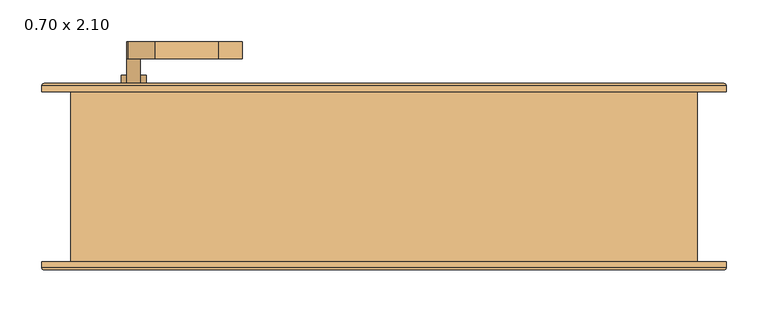
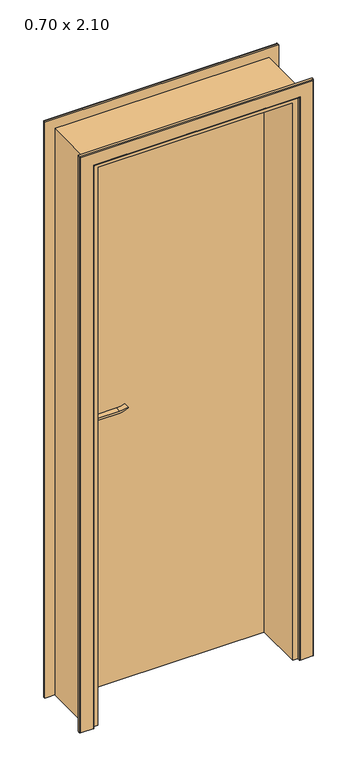
"""IFC4 building model written with IfcOpenShell, lengths in millimetres: door geometry, .CC_ND 300_PORTA SIMPLES DE ABRIR_COM EXTENSÃO : 0.70 x 2.10."""

from ifc_helpers import new_model, si_unit, point, frame, frame_2d, origin, origin_with_axes, place, context, project, spatial, polyline, circle_curve, ellipse_curve, trimmed, segment, composite_curve, outline, extrude, faceted_brep, source, transform, mapped, element, save
from ifc_brep_helpers import plane_surface, cylinder_surface, advanced_brep


def door_0_70_x_2_10_de0bd01c(model_context):
    return source(origin(), model_context, "Body", "SolidModel", [
        extrude(outline(composite_curve([segment(trimmed(circle_curve(frame_2d((964.5, -300.0)), 15.0), [point((964.5, -285.0))], [point((964.5, -315.0))], False, "CARTESIAN"), True, "CONTINUOUS"), segment(trimmed(circle_curve(frame_2d((964.5, -300.0)), 15.0), [point((964.5, -315.0))], [point((964.5, -285.0))], False, "CARTESIAN"), True, "CONTINUOUS")], self_intersect=False)), frame((0.0, 126.4, 0.0), z_axis=(0.0, 1.0, 0.0), x_axis=(0.0, 0.0, 1.0)), (0.0, 0.0, 1.0), 10.0),
        extrude(outline(composite_curve([segment(trimmed(circle_curve(frame_2d((964.5, -300.0)), 15.0), [point((964.5, -285.0))], [point((964.5, -315.0))], False, "CARTESIAN"), True, "CONTINUOUS"), segment(trimmed(circle_curve(frame_2d((964.5, -300.0)), 15.0), [point((964.5, -315.0))], [point((964.5, -285.0))], False, "CARTESIAN"), True, "CONTINUOUS")], self_intersect=False)), frame((0.0, 66.4, 0.0), z_axis=(0.0, 1.0, 0.0), x_axis=(0.0, 0.0, 1.0)), (0.0, 0.0, 1.0), 10.0),
        extrude(outline(composite_curve([segment(trimmed(circle_curve(frame_2d((1024.5, -300.0)), 8.0), [point((1029.1523287, -306.5081363))], [point((1024.5, -292.0))], False, "CARTESIAN"), True, "CONTINUOUS"), segment(trimmed(circle_curve(frame_2d((1019.3738613, -274.6138099)), 18.1261387), [point((1024.5, -292.0))], [point((1037.5, -274.6138099))], True, "CARTESIAN"), True, "CONTINUOUS"), segment(polyline([(1037.5, -274.6138099), (1037.5, -198.3564091)]), True, "CONTINUOUS"), segment(trimmed(circle_curve(frame_2d((1096.7709207, -201.9396612)), 59.3791355), [point((1037.5, -198.3564091))], [point((1046.7135558, -170.0))], False, "CARTESIAN"), True, "CONTINUOUS"), segment(polyline([(1046.7135558, -170.0), (1049.5, -170.0)]), True, "CONTINUOUS"), segment(trimmed(circle_curve(frame_2d((1127.7850638, -198.4227909)), 83.2850902), [point((1049.5, -170.0))], [point((1044.5, -198.3564091))], True, "CARTESIAN"), True, "CONTINUOUS"), segment(polyline([(1044.5, -198.3564091), (1044.5, -274.6325667)]), True, "CONTINUOUS"), segment(trimmed(circle_curve(frame_2d((1007.2555521, -276.3324871)), 37.2832219), [point((1044.5, -274.6325667))], [point((1029.1523287, -306.5081363))], False, "CARTESIAN"), True, "CONTINUOUS")], self_intersect=False)), frame((0.0, 156.4, 0.0), z_axis=(0.0, 1.0, 0.0), x_axis=(0.0, 0.0, 1.0)), (0.0, 0.0, 1.0), 20.0),
        extrude(outline(composite_curve([segment(trimmed(circle_curve(frame_2d((1019.3738682, -274.6138122)), 18.1261318), [point((1024.4999903, -292.0))], [point((1037.5, -274.6138122))], True, "CARTESIAN"), True, "CONTINUOUS"), segment(polyline([(1037.5, -274.6138122), (1037.5, -198.3564091)]), True, "CONTINUOUS"), segment(trimmed(circle_curve(frame_2d((1096.7709207, -201.9396612)), 59.3791355), [point((1037.5, -198.3564091))], [point((1046.7135558, -170.0))], False, "CARTESIAN"), True, "CONTINUOUS"), segment(polyline([(1046.7135558, -170.0), (1049.5, -170.0)]), True, "CONTINUOUS"), segment(trimmed(circle_curve(frame_2d((1127.7850638, -198.4227909)), 83.2850902), [point((1049.5, -170.0))], [point((1044.5, -198.3564091))], True, "CARTESIAN"), True, "CONTINUOUS"), segment(polyline([(1044.5, -198.3564091), (1044.5, -274.6325667)]), True, "CONTINUOUS"), segment(trimmed(circle_curve(frame_2d((1007.2555521, -276.3324871)), 37.2832219), [point((1044.5, -274.6325667))], [point((1029.1523287, -306.5081363))], False, "CARTESIAN"), True, "CONTINUOUS"), segment(trimmed(circle_curve(frame_2d((1024.5, -300.0)), 8.0), [point((1029.1523287, -306.5081363))], [point((1024.4999903, -292.0))], False, "CARTESIAN"), True, "CONTINUOUS")], self_intersect=False)), frame((0.0, 26.4, 0.0), z_axis=(0.0, 1.0, 0.0), x_axis=(0.0, 0.0, 1.0)), (0.0, 0.0, 1.0), 20.0),
        extrude(outline(composite_curve([segment(trimmed(circle_curve(frame_2d((1024.5, -300.0)), 8.0), [point((1024.5, -292.0))], [point((1024.5, -308.0))], False, "CARTESIAN"), True, "CONTINUOUS"), segment(trimmed(circle_curve(frame_2d((1024.5, -300.0)), 8.0), [point((1024.5, -308.0))], [point((1024.5, -292.0))], False, "CARTESIAN"), True, "CONTINUOUS")], self_intersect=False)), frame((0.0, 126.4, 0.0), z_axis=(0.0, 1.0, 0.0), x_axis=(0.0, 0.0, 1.0)), (0.0, 0.0, 1.0), 30.0),
        extrude(outline(composite_curve([segment(trimmed(circle_curve(frame_2d((1024.5, -300.0)), 8.0), [point((1024.5, -292.0))], [point((1024.5, -308.0))], False, "CARTESIAN"), True, "CONTINUOUS"), segment(trimmed(circle_curve(frame_2d((1024.5, -300.0)), 8.0), [point((1024.5, -308.0))], [point((1024.5, -292.0))], False, "CARTESIAN"), True, "CONTINUOUS")], self_intersect=False)), frame((0.0, 46.4, 0.0), z_axis=(0.0, 1.0, 0.0), x_axis=(0.0, 0.0, 1.0)), (0.0, 0.0, 1.0), 30.0),
        extrude(outline(composite_curve([segment(trimmed(circle_curve(frame_2d((954.5, -300.0)), 25.0), [point((954.5, -325.0))], [point((954.5, -275.0))], False, "CARTESIAN"), True, "CONTINUOUS"), segment(polyline([(954.5, -275.0), (1024.5, -275.0)]), True, "CONTINUOUS"), segment(trimmed(circle_curve(frame_2d((1024.5, -300.0)), 25.0), [point((1024.5, -275.0))], [point((1024.5, -325.0))], False, "CARTESIAN"), True, "CONTINUOUS"), segment(polyline([(1024.5, -325.0), (954.5, -325.0)]), True, "CONTINUOUS")], self_intersect=False)), frame((0.0, 116.4, 0.0), z_axis=(0.0, 1.0, 0.0), x_axis=(0.0, 0.0, 1.0)), (0.0, 0.0, 1.0), 10.0),
        extrude(outline(composite_curve([segment(trimmed(circle_curve(frame_2d((954.5, -300.0)), 25.0), [point((954.5, -325.0))], [point((954.5, -275.0))], False, "CARTESIAN"), True, "CONTINUOUS"), segment(polyline([(954.5, -275.0), (1024.5, -275.0)]), True, "CONTINUOUS"), segment(trimmed(circle_curve(frame_2d((1024.5, -300.0)), 25.0), [point((1024.5, -275.0))], [point((1024.5, -325.0))], False, "CARTESIAN"), True, "CONTINUOUS"), segment(polyline([(1024.5, -325.0), (954.5, -325.0)]), True, "CONTINUOUS")], self_intersect=False)), frame((0.0, 76.4, 0.0), z_axis=(0.0, 1.0, 0.0), x_axis=(0.0, 0.0, 1.0)), (0.0, 0.0, 1.0), 10.0),
        advanced_brep(
        [(-410.0, 116.4, 0.0), (-410.0, 123.4, 0.0), (-407.0, 126.4, 0.0), (-363.0, 126.4, 0.0), (-360.0, 123.4, 0.0), (-360.0, 116.4, 0.0), (-360.0, 116.4, 2085.0), (360.0, 116.4, 2085.0), (360.0, 116.4, 0.0), (410.0, 116.4, 0.0), (410.0, 116.4, 2135.0), (-410.0, 116.4, 2135.0), (-360.0, 123.4, 2085.0), (-363.0, 126.4, 2088.0), (-407.0, 126.4, 2132.0), (407.0, 126.4, 2132.0), (407.0, 126.4, 0.0), (363.0, 126.4, 0.0), (363.0, 126.4, 2088.0), (-410.0, 123.4, 2135.0), (410.0, 123.4, 0.0), (410.0, 123.4, 2135.0), (360.0, 123.4, 0.0), (360.0, 123.4, 2085.0)],
        [
            (0, 1),
            (1, 2, circle_curve(frame((-407.0, 123.4, 0.0), z_axis=(0.0, 0.0, -1.0), x_axis=(1.0, 0.0, 0.0)), 3.0)),
            (2, 3),
            (3, 4, circle_curve(frame((-363.0, 123.4, 0.0), z_axis=(0.0, 0.0, -1.0), x_axis=(1.0, 0.0, 0.0)), 3.0)),
            (4, 5),
            (5, 0),
            (5, 6),
            (6, 7),
            (7, 8),
            (8, 9),
            (9, 10),
            (10, 11),
            (11, 0),
            (4, 12),
            (12, 6),
            (3, 13),
            (13, 12, ellipse_curve(frame((-363.0, 123.4, 2088.0), z_axis=(-0.7071067811865475, 0.0, -0.7071067811865475), x_axis=(0.7071067811865474, 0.0, -0.7071067811865476)), 4.2426407, 3.0)),
            (2, 14),
            (14, 15),
            (15, 16),
            (16, 17),
            (17, 18),
            (18, 13),
            (1, 19),
            (19, 14, ellipse_curve(frame((-407.0, 123.4, 2132.0), z_axis=(-0.7071067811865475, 0.0, -0.7071067811865475), x_axis=(0.7071067811865474, 0.0, -0.7071067811865476)), 4.2426407, 3.0)),
            (11, 19),
            (9, 20),
            (20, 21),
            (21, 10),
            (8, 22),
            (22, 17, circle_curve(frame((363.0, 123.4, 0.0), z_axis=(0.0, 0.0, -1.0), x_axis=(-1.0, 0.0, 0.0)), 3.0)),
            (16, 20, circle_curve(frame((407.0, 123.4, 0.0), z_axis=(0.0, 0.0, -1.0), x_axis=(-1.0, 0.0, 0.0)), 3.0)),
            (23, 22),
            (7, 23),
            (23, 18, ellipse_curve(frame((363.0, 123.4, 2088.0), z_axis=(0.7071067811865475, 0.0, -0.7071067811865475), x_axis=(0.7071067811865474, 0.0, 0.7071067811865476)), 4.2426407, 3.0)),
            (15, 21, ellipse_curve(frame((407.0, 123.4, 2132.0), z_axis=(0.7071067811865475, 0.0, -0.7071067811865475), x_axis=(0.7071067811865474, 0.0, 0.7071067811865476)), 4.2426407, 3.0)),
            (12, 23),
            (21, 19),
        ],
        [
            plane_surface(frame((-360.0, 116.4, 0.0), z_axis=(0.0, 0.0, -1.0), x_axis=(0.0, -1.0, 0.0))),
            plane_surface(frame((-410.0, 116.4, 0.0), z_axis=(0.0, -1.0, 0.0), x_axis=(0.0, 0.0, 1.0))),
            plane_surface(frame((-360.0, 116.4, 0.0), z_axis=(1.0, 0.0, 0.0), x_axis=(0.0, 0.0, 1.0))),
            cylinder_surface(frame((-363.0, 123.4, 0.0), z_axis=(0.0, 0.0, -1.0), x_axis=(1.0, 0.0, 0.0)), 3.0),
            plane_surface(frame((-363.0, 126.4, 0.0), z_axis=(0.0, 1.0, 0.0), x_axis=(0.0, 0.0, 1.0))),
            cylinder_surface(frame((-407.0, 123.4, 0.0), z_axis=(0.0, 0.0, -1.0), x_axis=(1.0, 0.0, 0.0)), 3.0),
            plane_surface(frame((-410.0, 123.4, 0.0), z_axis=(-1.0, 0.0, 0.0), x_axis=(0.0, 0.0, 1.0))),
            plane_surface(frame((410.0, 123.4, 2135.0), z_axis=(1.0, 0.0, 0.0), x_axis=(0.0, 0.0, -1.0))),
            plane_surface(frame((360.0, 116.4, 0.0), z_axis=(0.0, 0.0, -1.0), x_axis=(0.0, -1.0, 0.0))),
            plane_surface(frame((360.0, 116.4, 2085.0), z_axis=(-1.0, 0.0, 0.0), x_axis=(0.0, 0.0, -1.0))),
            cylinder_surface(frame((363.0, 123.4, 2085.0), z_axis=(0.0, 0.0, 1.0), x_axis=(-1.0, 0.0, 0.0)), 3.0),
            cylinder_surface(frame((407.0, 123.4, 2085.0), z_axis=(0.0, 0.0, 1.0), x_axis=(-1.0, 0.0, 0.0)), 3.0),
            plane_surface(frame((-360.0, 116.4, 2085.0), z_axis=(0.0, 0.0, -1.0), x_axis=(1.0, 0.0, 0.0))),
            plane_surface(frame((-410.0, 123.4, 2135.0), z_axis=(0.0, 0.0, 1.0), x_axis=(1.0, 0.0, 0.0))),
            cylinder_surface(frame((-360.0, 123.4, 2088.0), z_axis=(-1.0, 0.0, 0.0), x_axis=(0.0, 0.0, -1.0)), 3.0),
            cylinder_surface(frame((-360.0, 123.4, 2132.0), z_axis=(-1.0, 0.0, 0.0), x_axis=(0.0, 0.0, -1.0)), 3.0),
        ],
        [
            (0, [[1, 2, 3, 4, 5, 6]]),
            (1, [[7, 8, 9, 10, 11, 12, 13, -6]]),
            (2, [[14, 15, -7, -5]]),
            (3, [[16, 17, -14, -4]]),
            (4, [[18, 19, 20, 21, 22, 23, -16, -3]]),
            (5, [[24, 25, -18, -2]]),
            (6, [[-13, 26, -24, -1]]),
            (7, [[-11, 27, 28, 29]]),
            (8, [[-10, 30, 31, -21, 32, -27]]),
            (9, [[33, -30, -9, 34]]),
            (10, [[-22, -31, -33, 35]]),
            (11, [[-28, -32, -20, 36]]),
            (12, [[37, -34, -8, -15]]),
            (13, [[-12, -29, 38, -26]]),
            (14, [[-23, -35, -37, -17]]),
            (15, [[-38, -36, -19, -25]]),
        ],
    ),
        advanced_brep(
        [(410.0, -86.9, 0.0), (410.0, -93.9342217, 0.0), (407.0342217, -96.9, 0.0), (362.9842717, -96.9, 0.0), (360.0, -93.9157283, 0.0), (360.0, -86.9, 0.0), (360.0, -86.9, 2085.0), (-360.0, -86.9, 2085.0), (-360.0, -86.9, 0.0), (-410.0, -86.9, 0.0), (-410.0, -86.9, 2135.0), (410.0, -86.9, 2135.0), (360.0, -93.9157283, 2085.0), (362.9842717, -96.9, 2087.9842717), (407.0342217, -96.9, 2132.0342217), (-407.0342217, -96.9, 2132.0342217), (-407.0342217, -96.9, 0.0), (-362.9842717, -96.9, 0.0), (-362.9842717, -96.9, 2087.9842717), (410.0, -93.9342217, 2135.0), (-410.0, -93.9342217, 0.0), (-410.0, -93.9342217, 2135.0), (-360.0, -93.9157283, 0.0), (-360.0, -93.9157283, 2085.0)],
        [
            (0, 1),
            (1, 2, circle_curve(frame((407.0342217, -93.9342217, 0.0), z_axis=(0.0, 0.0, -1.0), x_axis=(1.0, 0.0, 0.0)), 2.9657783)),
            (2, 3),
            (3, 4, circle_curve(frame((362.9842717, -93.9157283, 0.0), z_axis=(0.0, 0.0, -1.0), x_axis=(1.0, 0.0, 0.0)), 2.9842717)),
            (4, 5),
            (5, 0),
            (5, 6),
            (6, 7),
            (7, 8),
            (8, 9),
            (9, 10),
            (10, 11),
            (11, 0),
            (4, 12),
            (12, 6),
            (3, 13),
            (13, 12, ellipse_curve(frame((362.9842717, -93.9157283, 2087.9842717), z_axis=(0.7071067811865475, 0.0, -0.7071067811865475), x_axis=(-0.7071067811865474, 0.0, -0.7071067811865476)), 4.2203975, 2.9842717)),
            (2, 14),
            (14, 15),
            (15, 16),
            (16, 17),
            (17, 18),
            (18, 13),
            (1, 19),
            (19, 14, ellipse_curve(frame((407.0342217, -93.9342217, 2132.0342217), z_axis=(0.7071067811865475, 0.0, -0.7071067811865475), x_axis=(-0.7071067811865474, 0.0, -0.7071067811865476)), 4.1942438, 2.9657783)),
            (11, 19),
            (9, 20),
            (20, 21),
            (21, 10),
            (8, 22),
            (22, 17, circle_curve(frame((-362.9842717, -93.9157283, 0.0), z_axis=(0.0, 0.0, -1.0), x_axis=(-1.0, 0.0, 0.0)), 2.9842717)),
            (16, 20, circle_curve(frame((-407.0342217, -93.9342217, 0.0), z_axis=(0.0, 0.0, -1.0), x_axis=(-1.0, 0.0, 0.0)), 2.9657783)),
            (23, 22),
            (7, 23),
            (23, 18, ellipse_curve(frame((-362.9842717, -93.9157283, 2087.9842717), z_axis=(-0.7071067811865475, 0.0, -0.7071067811865475), x_axis=(-0.7071067811865474, 0.0, 0.7071067811865476)), 4.2203975, 2.9842717)),
            (15, 21, ellipse_curve(frame((-407.0342217, -93.9342217, 2132.0342217), z_axis=(-0.7071067811865475, 0.0, -0.7071067811865475), x_axis=(-0.7071067811865474, 0.0, 0.7071067811865476)), 4.1942438, 2.9657783)),
            (12, 23),
            (21, 19),
        ],
        [
            plane_surface(frame((360.0, -86.9, 0.0), z_axis=(0.0, 0.0, -1.0), x_axis=(0.0, -1.0, 0.0))),
            plane_surface(frame((410.0, -86.9, 0.0), z_axis=(0.0, 1.0, 0.0), x_axis=(0.0, 0.0, 1.0))),
            plane_surface(frame((360.0, -86.9, 0.0), z_axis=(-1.0, 0.0, 0.0), x_axis=(0.0, 0.0, 1.0))),
            cylinder_surface(frame((362.9842717, -93.9157283, 0.0), z_axis=(0.0, 0.0, -1.0), x_axis=(1.0, 0.0, 0.0)), 2.9842717),
            plane_surface(frame((362.9842717, -96.9, 0.0), z_axis=(0.0, -1.0, 0.0), x_axis=(0.0, 0.0, 1.0))),
            cylinder_surface(frame((407.0342217, -93.9342217, 0.0), z_axis=(0.0, 0.0, -1.0), x_axis=(1.0, 0.0, 0.0)), 2.9657783),
            plane_surface(frame((410.0, -93.9342217, 0.0), z_axis=(1.0, 0.0, 0.0), x_axis=(0.0, 0.0, 1.0))),
            plane_surface(frame((-410.0, -93.9342217, 2135.0), z_axis=(-1.0, 0.0, 0.0), x_axis=(0.0, 0.0, -1.0))),
            plane_surface(frame((-360.0, -86.9, 0.0), z_axis=(0.0, 0.0, -1.0), x_axis=(0.0, -1.0, 0.0))),
            plane_surface(frame((-360.0, -86.9, 2085.0), z_axis=(1.0, 0.0, 0.0), x_axis=(0.0, 0.0, -1.0))),
            cylinder_surface(frame((-362.9842717, -93.9157283, 2085.0), z_axis=(0.0, 0.0, 1.0), x_axis=(-1.0, 0.0, 0.0)), 2.9842717),
            cylinder_surface(frame((-407.0342217, -93.9342217, 2085.0), z_axis=(0.0, 0.0, 1.0), x_axis=(-1.0, 0.0, 0.0)), 2.9657783),
            plane_surface(frame((360.0, -86.9, 2085.0), z_axis=(0.0, 0.0, -1.0), x_axis=(-1.0, 0.0, 0.0))),
            plane_surface(frame((410.0, -93.9342217, 2135.0), z_axis=(0.0, 0.0, 1.0), x_axis=(-1.0, 0.0, 0.0))),
            cylinder_surface(frame((360.0, -93.9157283, 2087.9842717), z_axis=(1.0, 0.0, 0.0), x_axis=(0.0, 0.0, 1.0)), 2.9842717),
            cylinder_surface(frame((360.0, -93.9342217, 2132.0342217), z_axis=(1.0, 0.0, 0.0), x_axis=(0.0, 0.0, 1.0)), 2.9657783),
        ],
        [
            (0, [[1, 2, 3, 4, 5, 6]]),
            (1, [[7, 8, 9, 10, 11, 12, 13, -6]]),
            (2, [[14, 15, -7, -5]]),
            (3, [[16, 17, -14, -4]]),
            (4, [[18, 19, 20, 21, 22, 23, -16, -3]]),
            (5, [[24, 25, -18, -2]]),
            (6, [[-13, 26, -24, -1]]),
            (7, [[-11, 27, 28, 29]]),
            (8, [[-10, 30, 31, -21, 32, -27]]),
            (9, [[33, -30, -9, 34]]),
            (10, [[-22, -31, -33, 35]]),
            (11, [[-28, -32, -20, 36]]),
            (12, [[37, -34, -8, -15]]),
            (13, [[-12, -29, 38, -26]]),
            (14, [[-23, -35, -37, -17]]),
            (15, [[-38, -36, -19, -25]]),
        ],
    ),
        faceted_brep([(342.0, -86.9, 0.0), (342.0, 86.4, 0.0), (350.0, 86.4, 0.0), (350.0, 116.4, 0.0), (375.0, 116.4, 0.0), (375.0, -86.9, 0.0), (375.0, -86.9, 2100.0), (-375.0, -86.9, 2100.0), (-375.0, -86.9, 0.0), (-342.0, -86.9, 0.0), (-342.0, -86.9, 2067.0), (342.0, -86.9, 2067.0), (375.0, 116.4, 2100.0), (350.0, 116.4, 2075.0), (-350.0, 116.4, 2075.0), (-350.0, 116.4, 0.0), (-375.0, 116.4, 0.0), (-375.0, 116.4, 2100.0), (350.0, 86.4, 2075.0), (342.0, 86.4, 2067.0), (-342.0, 86.4, 2067.0), (-342.0, 86.4, 0.0), (-350.0, 86.4, 0.0), (-350.0, 86.4, 2075.0)], [[[0, 1, 2, 3, 4, 5]], [[5, 6, 7, 8, 9, 10, 11, 0]], [[4, 12, 6, 5]], [[3, 13, 14, 15, 16, 17, 12, 4]], [[2, 18, 13, 3]], [[1, 19, 20, 21, 22, 23, 18, 2]], [[0, 11, 19, 1]], [[10, 9, 21, 20]], [[9, 8, 16, 15, 22, 21]], [[17, 16, 8, 7]], [[23, 22, 15, 14]], [[12, 17, 7, 6]], [[18, 23, 14, 13]], [[11, 10, 20, 19]]]),
        extrude(outline(polyline([(-350.0, 86.4), (-350.0, 116.4), (350.0, 116.4), (350.0, 86.4), (-350.0, 86.4)])), origin_with_axes(), (0.0, 0.0, 1.0), 2075.0),
    ])


if __name__ == "__main__":
    model = new_model("IFC4")
    model_context = context("Model", 3, world=origin())
    ifc_project = project(units=[si_unit("LENGTHUNIT", "METRE", prefix="MILLI")], contexts=[model_context])
    site = spatial("IfcSite", under=ifc_project)
    building = spatial("IfcBuilding", under=site)
    placement = place(None, origin())
    door_0_70_x_2_10_shape = door_0_70_x_2_10_de0bd01c(model_context)
    element("IfcDoor", 1, ObjectType=".CC_ND 300_PORTA SIMPLES DE ABRIR_COM EXTENSÃO : 0.70 x 2.10", at=placement, inside=building, context=model_context, shape_type="MappedRepresentation", body=[
        mapped(door_0_70_x_2_10_shape, transform((0.0, 0.0, 0.0), x_axis=(1.0, 0.0, 0.0), y_axis=(0.0, 1.0, 0.0), z_axis=(0.0, 0.0, 1.0))),
    ])
    save(model, "model.ifc")

# Revit data of these elements
# Type ".CC_ND 300_PORTA SIMPLES DE ABRIR_COM EXTENSÃO : 0.70 x 2.10"
#   Type Mark = "155"
#   Rough Width = 0.75 m
#   Espessura moldura externa = 0.01 m
#   Espessura moldura interna = 0.01 m
#   Largura moldura = 0.05 m
#   Extensão acabamento exterior [instance default] = 0.00 m
#   Extensão acabamento interior [instance default] = 0.00 m
#   Espessura batente = 0.025 m
#   Thickness = 0.03 m
#   Altura batente = 2.085 m
#   Aux Arco [instance default] = 0.70 m
#   Rough Height = 2.125 m
#   Height = 2.10 m
#   Width = 0.70 m
#   Moldura interna [instance default] = yes
#   Moldura externa [instance default] = yes
#   Porta = .MADEIRA COM PINTURA ESMALTE BRANCO ACETINADO
#   Moldura = .MADEIRA COM PINTURA ESMALTE BRANCO ACETINADO
#   Maçaneta = .ALUMÍNIO
#   Batente = .MADEIRA COM PINTURA ESMALTE BRANCO ACETINADO
#   Function = (empty or 0)
#   Wall Closure = (empty or 0)
# Element 1 (IfcDoor, ".CC_ND 300_PORTA SIMPLES DE ABRIR_COM EXTENSÃO : 0.70 x 2.10")
#   Extensão acabamento interior = 0.0295 m
#   Aux Arco = 0.7295 m
#   Materials on its faces: ".MADEIRA COM PINTURA ESMALTE BRANCO ACETINADO", ".ALUMÍNIO"
# Materials
#   ".MADEIRA COM PINTURA ESMALTE BRANCO ACETINADO": class ".CC_MADEIRAS", colour RGB 240 240 240, transparency 0, Description = "Madeira com pintura esmalte branco acetinado.", Cost = 0
#   ".ALUMÍNIO": class "CC_METAIS", colour RGB 244 244 244, transparency 0, Description = "Material alumínio", Cost = 0
